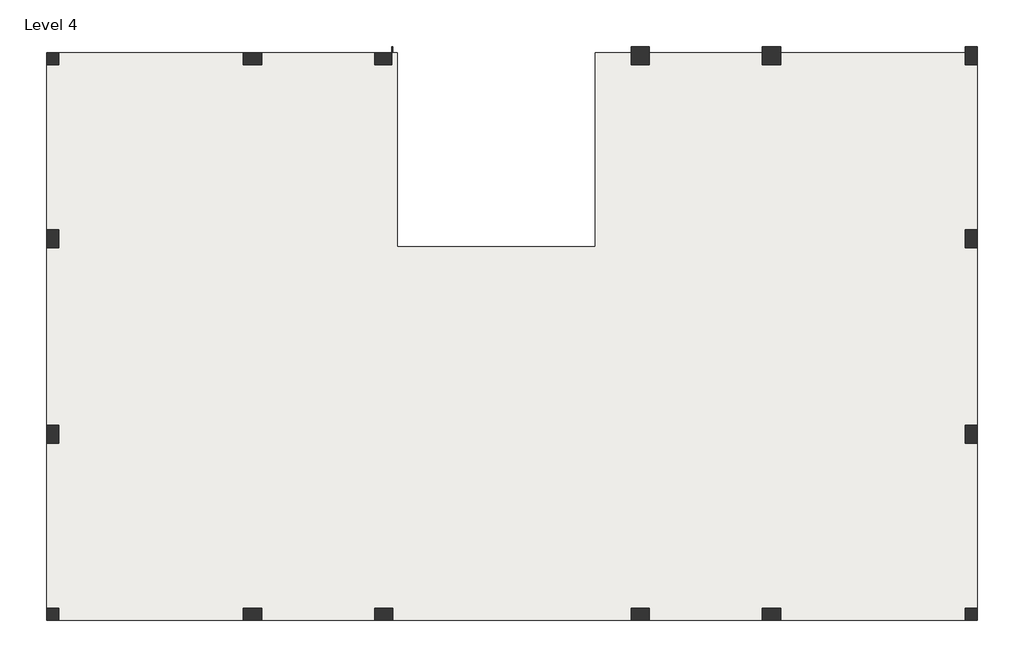
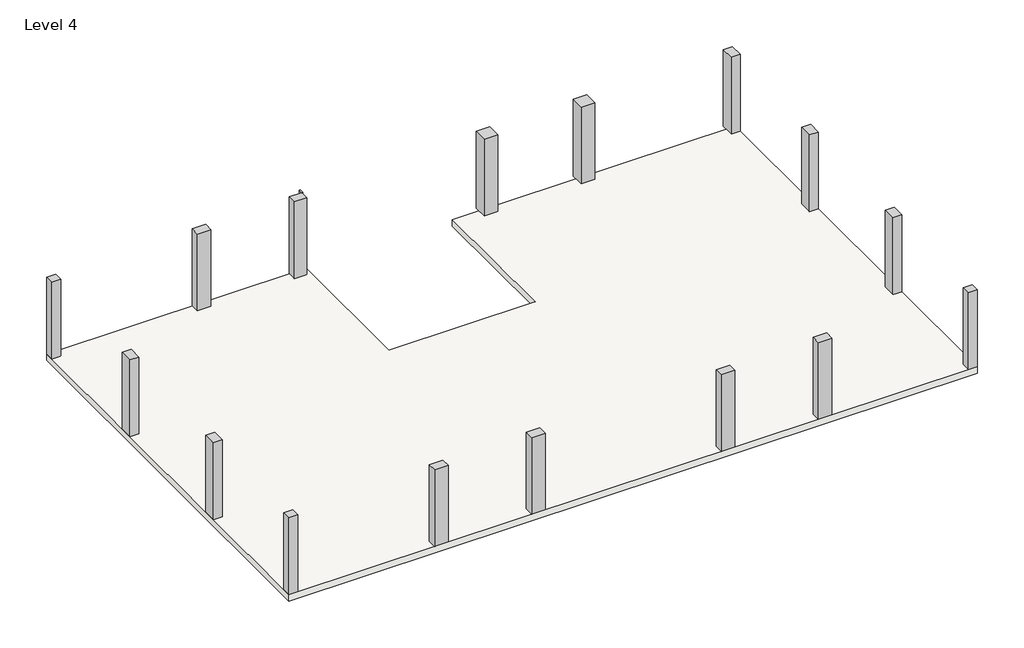
# One storey: 16 columns, 1 slab.
"""IFC4 building model written with IfcOpenShell, lengths in millimetres."""

import ifcopenshell
import ifcopenshell.guid

model = None  # the IFC model being written
_history = None  # IfcOwnerHistory: only IFC2X3 demands one
_inside = {}  # id of a spatial element -> (the spatial element, [elements in it])
_under = {}  # id of a project, library or spatial element -> (it, [spatial elements below it])
_declared = {}  # id of a project -> (the project, [libraries it declares])
_typed = {}  # id of a type object -> (the type object, [elements of that type])
_made_of = {}  # id of a material, layer set ... -> (it, [elements and type objects made of it])


def new_model(schema):
    """Start an empty IFC model of exactly this schema.

    Asked for "IFC4X3", IfcOpenShell would pick the latest addendum, in which some entities
    have other attributes; the version numbers below select the first issue.
    IFC2X3 requires an IfcOwnerHistory on every rooted entity: one is made here for all.
    """
    global model, _history
    if schema == "IFC4X3":
        model = ifcopenshell.file(schema_version=(4, 3, 0, 0))
    else:
        model = ifcopenshell.file(schema=schema)
    _inside.clear()
    _under.clear()
    _declared.clear()
    _typed.clear()
    _made_of.clear()
    _history = None
    if model.schema == "IFC2X3":
        org = make("IfcOrganization", Name="unknown")
        user = make(
            "IfcPersonAndOrganization",
            ThePerson=make("IfcPerson", FamilyName="unknown"),
            TheOrganization=org,
        )
        app = make(
            "IfcApplication",
            ApplicationDeveloper=org,
            Version="unknown",
            ApplicationFullName="unknown",
            ApplicationIdentifier="unknown",
        )
        _history = make(
            "IfcOwnerHistory",
            OwningUser=user,
            OwningApplication=app,
            ChangeAction="ADDED",
            CreationDate=0,
        )
    return model


def make(cls, **values):
    """One entity of the class cls with the attributes given. An attribute that is None is left unset."""
    return model.create_entity(
        cls, **{name: value for name, value in values.items() if value is not None}
    )


def rooted(cls, **values):
    """An entity with a GlobalId (a new one), such as an element, a storey or a relation."""
    return make(cls, GlobalId=ifcopenshell.guid.new(), OwnerHistory=_history, **values)


def si_unit(unit_type, name, prefix=None):
    """IfcSIUnit, for example si_unit("LENGTHUNIT", "METRE", prefix="MILLI")."""
    return make("IfcSIUnit", UnitType=unit_type, Prefix=prefix, Name=name)


def assignment(units):
    """IfcUnitAssignment: the units of a project."""
    return None if units is None else make("IfcUnitAssignment", Units=units)


def point(xyz):
    """IfcCartesianPoint."""
    return None if xyz is None else make("IfcCartesianPoint", Coordinates=xyz)


def direction(xyz):
    """IfcDirection."""
    return None if xyz is None else make("IfcDirection", DirectionRatios=xyz)


def frame(location, z_axis=None, x_axis=None):
    """IfcAxis2Placement3D, a coordinate frame: its origin and axes. An axis left out is left unset."""
    return make(
        "IfcAxis2Placement3D",
        Location=point(location),
        Axis=direction(z_axis),
        RefDirection=direction(x_axis),
    )


def origin():
    """The frame at (0, 0, 0) with its axes left unset."""
    return frame((0.0, 0.0, 0.0))


def place(relative_to, where):
    """IfcLocalPlacement: puts the frame where relative to a parent placement (None: the world)."""
    return make(
        "IfcLocalPlacement", PlacementRelTo=relative_to, RelativePlacement=where
    )


def context(
    kind, dimensions, precision=None, world=None, true_north=None, identifier=None
):
    """IfcGeometricRepresentationContext, for example the 3D "Model" context."""
    return make(
        "IfcGeometricRepresentationContext",
        ContextIdentifier=identifier,
        ContextType=kind,
        CoordinateSpaceDimension=dimensions,
        Precision=precision,
        WorldCoordinateSystem=world,
        TrueNorth=true_north,
    )


def project(units=None, contexts=None):
    """IfcProject with its units and contexts."""
    return rooted(
        "IfcProject",
        Name="project",
        RepresentationContexts=contexts,
        UnitsInContext=assignment(units),
    )


def spatial(cls, under=None, at=None, **own):
    """A site, building, storey or space (cls), placed at a placement, below another one or the project."""
    s = rooted(cls, ObjectPlacement=at, **own)
    if under is not None:
        _under.setdefault(under.id(), (under, []))[1].append(s)
    return s


def polyline(points):
    """IfcPolyline through the points."""
    return make("IfcPolyline", Points=[point(p) for p in points])


def outline(outer, holes=None, kind="AREA"):
    """IfcArbitraryClosedProfileDef: a profile drawn as a closed curve; with holes, ...WithVoids."""
    if holes is None:
        return make("IfcArbitraryClosedProfileDef", ProfileType=kind, OuterCurve=outer)
    return make(
        "IfcArbitraryProfileDefWithVoids",
        ProfileType=kind,
        OuterCurve=outer,
        InnerCurves=holes,
    )


def extrude(swept, where, along, depth):
    """IfcExtrudedAreaSolid: the profile swept, set in the frame where, extruded along a direction by depth."""
    return make(
        "IfcExtrudedAreaSolid",
        SweptArea=swept,
        Position=where,
        ExtrudedDirection=direction(along),
        Depth=depth,
    )


def shape(context_of_items, identifier, shape_type, items):
    """IfcShapeRepresentation: the items that make up one representation, for example the "Body"."""
    return make(
        "IfcShapeRepresentation",
        ContextOfItems=context_of_items,
        RepresentationIdentifier=identifier,
        RepresentationType=shape_type,
        Items=items,
    )


def made_of(thing, what):
    """Note that an element or type object is made of a material, layer set ...; save() writes the relation."""
    if what is not None:
        _made_of.setdefault(what.id(), (what, []))[1].append(thing)
    return thing


def element(
    cls,
    number,
    at=None,
    inside=None,
    cuts=None,
    type_object=None,
    material=None,
    context=None,
    identifier="Body",
    shape_type=None,
    held_by="IfcProductDefinitionShape",
    body=None,
    shapes=None,
    **own,
):
    """One element of the class cls, such as IfcWall. Its Tag is "e" and its number.

    at: its placement. inside: the storey or other place that contains it. cuts: it is an
    opening in that element (IfcRelVoidsElement). A single representation is given by context,
    identifier, shape_type and body (its items); several are given by shapes. held_by: the class
    of the entity that holds the representations. save() writes the other relations.
    """
    e = rooted(cls, Tag="e%d" % number, ObjectPlacement=at, **own)
    if body is not None:
        shapes = [shape(context, identifier, shape_type, body)]
    if shapes is not None:
        e.Representation = make(held_by, Representations=shapes)
    if inside is not None:
        _inside.setdefault(inside.id(), (inside, []))[1].append(e)
    if cuts is not None:
        rooted(
            "IfcRelVoidsElement", RelatingBuildingElement=cuts, RelatedOpeningElement=e
        )
    if type_object is not None:
        _typed.setdefault(type_object.id(), (type_object, []))[1].append(e)
    return made_of(e, material)


def aggregate(whole, parts):
    """IfcRelAggregates: a whole, such as a stair, and the parts it consists of."""
    return rooted("IfcRelAggregates", RelatingObject=whole, RelatedObjects=parts)


def save(model, path):
    """Write the relations noted so far, then the file.

    IfcRelAggregates (storeys below a building ...), IfcRelContainedInSpatialStructure (elements
    in a storey), IfcRelDefinesByType, IfcRelAssociatesMaterial and IfcRelDeclares: one each for
    every whole, place, type object, material and project.
    """
    for whole, parts in _under.values():
        aggregate(whole, parts)
    for where, things in _inside.values():
        rooted(
            "IfcRelContainedInSpatialStructure",
            RelatedElements=things,
            RelatingStructure=where,
        )
    for kind, things in _typed.values():
        rooted("IfcRelDefinesByType", RelatedObjects=things, RelatingType=kind)
    for what, things in _made_of.values():
        rooted("IfcRelAssociatesMaterial", RelatedObjects=things, RelatingMaterial=what)
    for by, libraries in _declared.values():
        rooted("IfcRelDeclares", RelatingContext=by, RelatedDefinitions=libraries)
    model.write(path)


model = new_model("IFC4")

# Units and contexts
model_context = context("Model", 3, world=origin())
ifc_project = project(units=[si_unit("LENGTHUNIT", "METRE", prefix="MILLI")], contexts=[model_context])

# Site, building, storey
site = spatial("IfcSite", under=ifc_project)
building = spatial("IfcBuilding", under=site)
storey = spatial("IfcBuildingStorey", under=building, Name="Level 4", Elevation=10972.8)

# Columns
placement = place(None, origin())
element("IfcColumn", 1, ObjectType="Rectangular Column : 24\" x 24\"", at=placement, inside=storey, context=model_context, shape_type="SweptSolid", body=[
    extrude(outline(polyline([(-16253.4122732, 9291.5015304), (-16253.4122732, 8885.1015304), (-16659.8122732, 8885.1015304), (-16659.8122732, 9291.5015304), (-16253.4122732, 9291.5015304)])), frame((0.0, 0.0, 10972.8), z_axis=(0.0, 0.0, 1.0), x_axis=(1.0, 0.0, 0.0)), (0.0, 0.0, 1.0), 3657.6),
])
element("IfcColumn", 2, ObjectType="Rectangular Column : 24\" x 24\"", at=placement, inside=storey, context=model_context, shape_type="SweptSolid", body=[
    extrude(outline(polyline([(-16253.4122732, 3398.7015304), (-16253.4122732, 2789.1015304), (-16659.8122732, 2789.1015304), (-16659.8122732, 3398.7015304), (-16253.4122732, 3398.7015304)])), frame((0.0, 0.0, 10972.8), z_axis=(0.0, 0.0, 1.0), x_axis=(1.0, 0.0, 0.0)), (0.0, 0.0, 1.0), 3657.6),
])
element("IfcColumn", 3, ObjectType="Rectangular Column : 24\" x 24\"", at=placement, inside=storey, context=model_context, shape_type="SweptSolid", body=[
    extrude(outline(polyline([(-9497.0122732, 8885.1015304), (-10106.6122732, 8885.1015304), (-10106.6122732, 9291.5015304), (-9497.0122732, 9291.5015304), (-9497.0122732, 8885.1015304)])), frame((0.0, 0.0, 10972.8), z_axis=(0.0, 0.0, 1.0), x_axis=(1.0, 0.0, 0.0)), (0.0, 0.0, 1.0), 3657.6),
])
element("IfcColumn", 4, ObjectType="Rectangular Column : 24\" x 24\"", at=placement, inside=storey, context=model_context, shape_type="SweptSolid", body=[
    extrude(outline(polyline([(-5174.2497732, 9494.7015304), (-5128.2122732, 9494.7015304), (-5128.2122732, 9301.0265304), (-5174.2497732, 9301.0265304), (-5174.2497732, 9494.7015304)])), frame((0.0, 0.0, 10972.8), z_axis=(0.0, 0.0, 1.0), x_axis=(1.0, 0.0, 0.0)), (0.0, 0.0, 1.0), 3657.6),
    extrude(outline(polyline([(-5737.8122732, 8885.1015304), (-5737.8122732, 9291.5015304), (-5174.2497732, 9291.5015304), (-5174.2497732, 8885.1015304), (-5737.8122732, 8885.1015304)])), frame((0.0, 0.0, 10972.8), z_axis=(0.0, 0.0, 1.0), x_axis=(1.0, 0.0, 0.0)), (0.0, 0.0, 1.0), 3657.6),
])
element("IfcColumn", 5, ObjectType="Rectangular Column : 24\" x 24\"", at=placement, inside=storey, context=model_context, shape_type="SweptSolid", body=[
    extrude(outline(polyline([(3406.1877268, 9494.7015304), (3406.1877268, 8885.1015304), (2796.5877268, 8885.1015304), (2796.5877268, 9494.7015304), (3406.1877268, 9494.7015304)])), frame((0.0, 0.0, 10972.8), z_axis=(0.0, 0.0, 1.0), x_axis=(1.0, 0.0, 0.0)), (0.0, 0.0, 1.0), 3657.6),
])
element("IfcColumn", 6, ObjectType="Rectangular Column : 24\" x 24\"", at=placement, inside=storey, context=model_context, shape_type="SweptSolid", body=[
    extrude(outline(polyline([(7774.9877268, 9494.7015304), (7774.9877268, 8885.1015304), (7165.3877268, 8885.1015304), (7165.3877268, 9494.7015304), (7774.9877268, 9494.7015304)])), frame((0.0, 0.0, 10972.8), z_axis=(0.0, 0.0, 1.0), x_axis=(1.0, 0.0, 0.0)), (0.0, 0.0, 1.0), 3657.6),
])
element("IfcColumn", 7, ObjectType="Rectangular Column : 24\" x 24\"", at=placement, inside=storey, context=model_context, shape_type="SweptSolid", body=[
    extrude(outline(polyline([(13921.7877268, 8885.1015304), (13921.7877268, 9494.7015304), (14328.1877268, 9494.7015304), (14328.1877268, 8885.1015304), (13921.7877268, 8885.1015304)])), frame((0.0, 0.0, 10972.8), z_axis=(0.0, 0.0, 1.0), x_axis=(1.0, 0.0, 0.0)), (0.0, 0.0, 1.0), 3657.6),
])
element("IfcColumn", 8, ObjectType="Rectangular Column : 24\" x 24\"", at=placement, inside=storey, context=model_context, shape_type="SweptSolid", body=[
    extrude(outline(polyline([(13921.7877268, 2789.1015304), (13921.7877268, 3398.7015304), (14328.1877268, 3398.7015304), (14328.1877268, 2789.1015304), (13921.7877268, 2789.1015304)])), frame((0.0, 0.0, 10972.8), z_axis=(0.0, 0.0, 1.0), x_axis=(1.0, 0.0, 0.0)), (0.0, 0.0, 1.0), 3657.6),
])
element("IfcColumn", 9, ObjectType="Rectangular Column : 24\" x 24\"", at=placement, inside=storey, context=model_context, shape_type="SweptSolid", body=[
    extrude(outline(polyline([(13921.7877268, -3713.2984696), (13921.7877268, -3103.6984696), (14328.1877268, -3103.6984696), (14328.1877268, -3713.2984696), (13921.7877268, -3713.2984696)])), frame((0.0, 0.0, 10972.8), z_axis=(0.0, 0.0, 1.0), x_axis=(1.0, 0.0, 0.0)), (0.0, 0.0, 1.0), 3657.6),
])
element("IfcColumn", 10, ObjectType="Rectangular Column : 24\" x 24\"", at=placement, inside=storey, context=model_context, shape_type="SweptSolid", body=[
    extrude(outline(polyline([(13921.7877268, -9606.0984696), (13921.7877268, -9199.6984696), (14328.1877268, -9199.6984696), (14328.1877268, -9606.0984696), (13921.7877268, -9606.0984696)])), frame((0.0, 0.0, 10972.8), z_axis=(0.0, 0.0, 1.0), x_axis=(1.0, 0.0, 0.0)), (0.0, 0.0, 1.0), 3657.6),
])
element("IfcColumn", 11, ObjectType="Rectangular Column : 24\" x 24\"", at=placement, inside=storey, context=model_context, shape_type="SweptSolid", body=[
    extrude(outline(polyline([(7165.3877268, -9199.6984696), (7774.9877268, -9199.6984696), (7774.9877268, -9606.0984696), (7165.3877268, -9606.0984696), (7165.3877268, -9199.6984696)])), frame((0.0, 0.0, 10972.8), z_axis=(0.0, 0.0, 1.0), x_axis=(1.0, 0.0, 0.0)), (0.0, 0.0, 1.0), 3657.6),
])
element("IfcColumn", 12, ObjectType="Rectangular Column : 24\" x 24\"", at=placement, inside=storey, context=model_context, shape_type="SweptSolid", body=[
    extrude(outline(polyline([(2796.5877268, -9199.6984696), (3406.1877268, -9199.6984696), (3406.1877268, -9606.0984696), (2796.5877268, -9606.0984696), (2796.5877268, -9199.6984696)])), frame((0.0, 0.0, 10972.8), z_axis=(0.0, 0.0, 1.0), x_axis=(1.0, 0.0, 0.0)), (0.0, 0.0, 1.0), 3657.6),
])
element("IfcColumn", 13, ObjectType="Rectangular Column : 24\" x 24\"", at=placement, inside=storey, context=model_context, shape_type="SweptSolid", body=[
    extrude(outline(polyline([(-5737.8122732, -9199.6984696), (-5128.2122732, -9199.6984696), (-5128.2122732, -9606.0984696), (-5737.8122732, -9606.0984696), (-5737.8122732, -9199.6984696)])), frame((0.0, 0.0, 10972.8), z_axis=(0.0, 0.0, 1.0), x_axis=(1.0, 0.0, 0.0)), (0.0, 0.0, 1.0), 3657.6),
])
element("IfcColumn", 14, ObjectType="Rectangular Column : 24\" x 24\"", at=placement, inside=storey, context=model_context, shape_type="SweptSolid", body=[
    extrude(outline(polyline([(-10106.6122732, -9199.6984696), (-9497.0122732, -9199.6984696), (-9497.0122732, -9606.0984696), (-10106.6122732, -9606.0984696), (-10106.6122732, -9199.6984696)])), frame((0.0, 0.0, 10972.8), z_axis=(0.0, 0.0, 1.0), x_axis=(1.0, 0.0, 0.0)), (0.0, 0.0, 1.0), 3657.6),
])
element("IfcColumn", 15, ObjectType="Rectangular Column : 24\" x 24\"", at=placement, inside=storey, context=model_context, shape_type="SweptSolid", body=[
    extrude(outline(polyline([(-16659.8122732, -9199.6984696), (-16253.4122732, -9199.6984696), (-16253.4122732, -9606.0984696), (-16659.8122732, -9606.0984696), (-16659.8122732, -9199.6984696)])), frame((0.0, 0.0, 10972.8), z_axis=(0.0, 0.0, 1.0), x_axis=(1.0, 0.0, 0.0)), (0.0, 0.0, 1.0), 3657.6),
])
element("IfcColumn", 16, ObjectType="Rectangular Column : 24\" x 24\"", at=placement, inside=storey, context=model_context, shape_type="SweptSolid", body=[
    extrude(outline(polyline([(-16253.4122732, -3103.6984696), (-16253.4122732, -3713.2984696), (-16659.8122732, -3713.2984696), (-16659.8122732, -3103.6984696), (-16253.4122732, -3103.6984696)])), frame((0.0, 0.0, 10972.8), z_axis=(0.0, 0.0, 1.0), x_axis=(1.0, 0.0, 0.0)), (0.0, 0.0, 1.0), 3657.6),
])

# Slab
element("IfcSlab", 17, ObjectType="Generic - 12\"", at=placement, inside=storey, context=model_context, shape_type="SweptSolid", body=[
    extrude(outline(polyline([(14328.1877268, 9291.5015304), (14328.1877268, -9606.0984696), (-16659.8122732, -9606.0984696), (-16659.8122732, 9291.5015304), (-4980.5747732, 9291.5015304), (-4980.5747732, 2835.1390304), (1602.7877268, 2835.1390304), (1602.7877268, 9291.5015304), (14328.1877268, 9291.5015304)])), frame((0.0, 0.0, 10668.0), z_axis=(0.0, 0.0, 1.0), x_axis=(1.0, 0.0, 0.0)), (0.0, 0.0, 1.0), 304.8),
])

save(model, "model.ifc")

# Revit data of these elements
# Type "Rectangular Column : 24\" x 24\""
#   Assembly Code = "B1010200"
#   Depth = 2' - 0"
#   Offset Base = 0' - 0"
#   Offset Top = 0' - 0"
#   Width = 2' - 0"
#   Material = none
# Type "Generic - 12\""
#   Assembly Code = "B1010"
#   Function = 0
#   Layers, outside or top first: 1' - 0" no material (function 1)
# Elements 1, 2, 3, 4, 7, 8, 9, 10, 11, 12, 13, 14, 15, 16 (IfcColumn, "Rectangular Column : 24\" x 24\"")
#   Phase Created = New Construction
#   Materials on its faces: "Default Wall"
# Elements 5, 6 (IfcColumn, "Rectangular Column : 24\" x 24\"")
#   Phase Created = New Construction
# Element 17 (IfcSlab, "Generic - 12\"")
#   built-in parameter 1001955 = 1.5708 (stored number, unit not read)
#   Height Offset From Level = 0' - 0"
#   Phase Created = New Construction
#   Materials on its faces: "Default Floor"
# Materials
#   "Default Wall": class "Miscellaneous", colour RGB 128 128 128, transparency 0, Cost = 0
#   "Default Floor": class "Miscellaneous", colour RGB 128 128 128, transparency 0, Cost = 0
